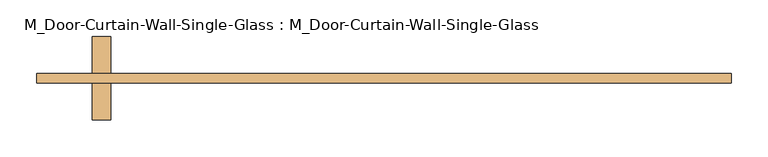
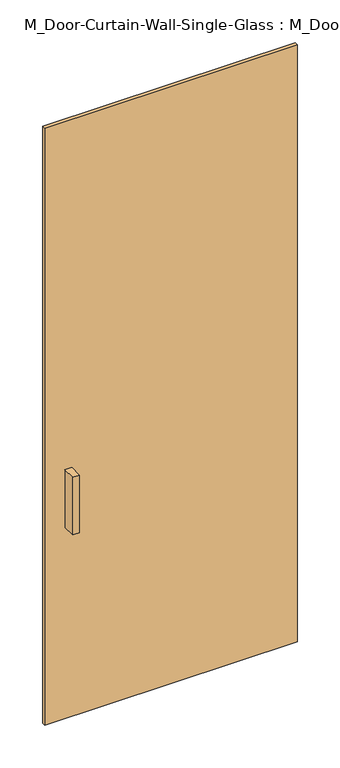
"""IFC4 building model written with IfcOpenShell, lengths in millimetres: door geometry, M_Door-Curtain-Wall-Single-Glass : M_Door-Curtain-Wall-Single-Glass."""

from ifc_helpers import new_model, si_unit, frame, origin, origin_with_axes, place, context, project, spatial, polyline, outline, extrude, source, transform, mapped, element, save


def m_door_curtain_wall_single_glass_m_door_curtain_wall_single_3c5a18a5(model_context):
    return source(origin(), model_context, "Body", "SweptSolid", [
        extrude(outline(polyline([(475.0, 50.8), (475.0, 38.1), (-475.0, 38.1), (-475.0, 50.8), (475.0, 50.8)])), origin_with_axes(), (0.0, 0.0, 1.0), 2375.0),
        extrude(outline(polyline([(-373.4, -12.7), (-398.8, -12.7), (-398.8, 38.1), (-373.4, 38.1), (-373.4, -12.7)])), frame((0.0, 0.0, 762.0), z_axis=(0.0, 0.0, 1.0), x_axis=(1.0, 0.0, 0.0)), (0.0, 0.0, 1.0), 228.6),
        extrude(outline(polyline([(-398.8, 101.6), (-373.4, 101.6), (-373.4, 50.8), (-398.8, 50.8), (-398.8, 101.6)])), frame((0.0, 0.0, 762.0), z_axis=(0.0, 0.0, 1.0), x_axis=(1.0, 0.0, 0.0)), (0.0, 0.0, 1.0), 228.6),
    ])


if __name__ == "__main__":
    model = new_model("IFC4")
    model_context = context("Model", 3, world=origin())
    ifc_project = project(units=[si_unit("LENGTHUNIT", "METRE", prefix="MILLI")], contexts=[model_context])
    site = spatial("IfcSite", under=ifc_project)
    building = spatial("IfcBuilding", under=site)
    placement = place(None, origin())
    m_door_curtain_wall_single_glass_m_door_curtain_wall_single_shape = m_door_curtain_wall_single_glass_m_door_curtain_wall_single_3c5a18a5(model_context)
    element("IfcDoor", 1, ObjectType="M_Door-Curtain-Wall-Single-Glass : M_Door-Curtain-Wall-Single-Glass", at=placement, inside=building, context=model_context, shape_type="MappedRepresentation", body=[
        mapped(m_door_curtain_wall_single_glass_m_door_curtain_wall_single_shape, transform((0.0, 0.0, 0.0), x_axis=(1.0, 0.0, 0.0), y_axis=(0.0, 1.0, 0.0), z_axis=(0.0, 0.0, 1.0))),
    ])
    save(model, "model.ifc")

# Revit data of these elements
# Type "M_Door-Curtain-Wall-Single-Glass : M_Door-Curtain-Wall-Single-Glass"
#   Type Mark = "50"
#   Assembly Code = "B2030100"
#   Analytic Construction = "<None>"
#   Width [instance default] = 900 mm
#   Thermal Resistance (R) = 1.7611 (m²·K)/W
#   Swing Angle [instance default] = 90.00°
#   Heat Transfer Coefficient (U) = 0.567826 W/(m²·K)
#   Offset = 50.8 mm
#   Define Thermal Properties by = 1
#   Function = 1
#   Door Handle Material = Aluminum
#   Glazing = Glass
#   Visual Light Transmittance = 0
#   Solar Heat Gain Coefficient = 0
#   Construction Type Id = ""
# Element 1 (IfcDoor, "M_Door-Curtain-Wall-Single-Glass : M_Door-Curtain-Wall-Single-Glass")
#   Width = 950 mm
#   Materials on its faces: "Aluminum", "Glass"
# Materials
#   "Aluminum": class "Metal", colour RGB 247 247 247, transparency 0, Description = "Aluminum 6061", Cost = 0
#   "Glass": class "Glass", colour RGB 0 128 192, transparency 0.9, Description = "Soda Lime Glass", Cost = 0
